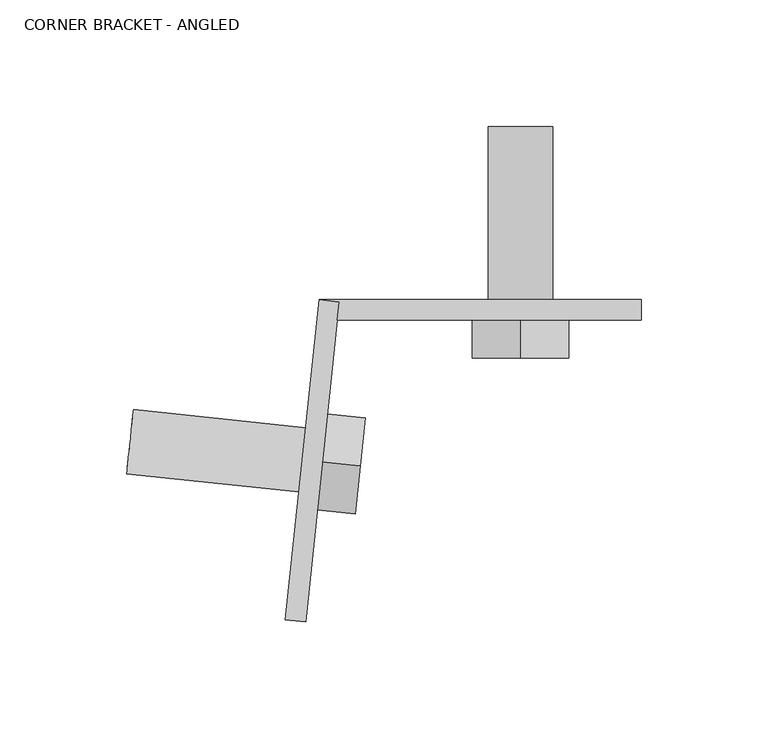
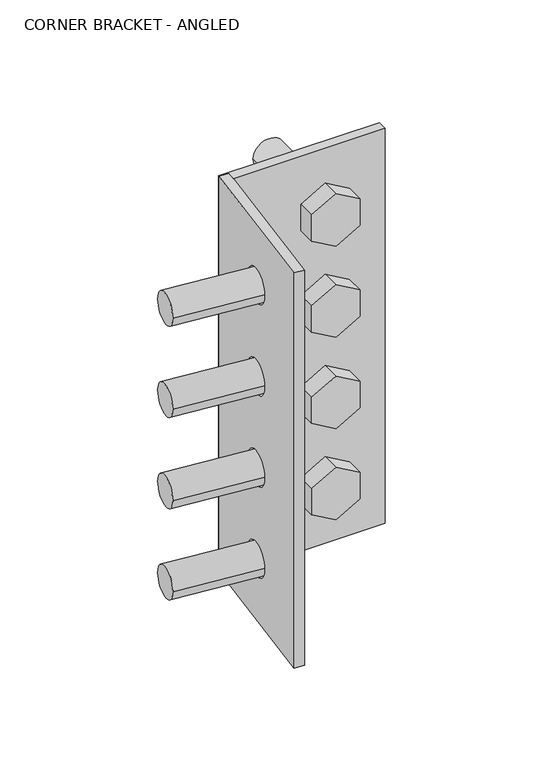
"""IFC4 building model written with IfcOpenShell, lengths in millimetres: fastener geometry, CORNER BRACKET - ANGLED."""

from ifc_helpers import new_model, si_unit, point, frame, frame_2d, origin, place, context, project, spatial, polyline, circle_curve, trimmed, segment, composite_curve, outline, extrude, source, transform, mapped, element, save
from ifc_brep_helpers import plane_surface, revolved_surface, advanced_brep


def corner_bracket_angled_dba65dea(model_context):
    return source(origin(), model_context, "Body", "SolidModel", [
        advanced_brep(
        [(65.484375, -7.9375, 203.2), (65.484375, 0.0, 203.2), (93.265625, 0.0, 203.2), (93.265625, -7.9375, 203.2), (93.265625, -7.9375, 279.4), (93.265625, 0.0, 279.4), (65.484375, 0.0, 279.4), (65.484375, -7.9375, 279.4), (127.0, 0.0, 0.0), (127.0, 0.0, 330.2), (127.0, -7.9375, 330.2), (127.0, -7.9375, 0.0), (65.484375, -7.9375, 127.0), (65.484375, 0.0, 127.0), (93.265625, 0.0, 127.0), (93.265625, -7.9375, 127.0), (65.484375, -7.9375, 50.8), (65.484375, 0.0, 50.8), (93.265625, 0.0, 50.8), (93.265625, -7.9375, 50.8), (7.1469571, -7.9375, 330.2), (7.1469571, -7.9375, 0.0), (0.0, 0.0, 0.0), (0.0, 0.0, 330.2), (7.8940175, -0.8296947, 330.2), (7.8940175, -0.8296947, 0.0)],
        [
            (0, 1),
            (1, 2, circle_curve(frame((79.375, 0.0, 203.2), z_axis=(0.0, 1.0, 0.0), x_axis=(-1.0000000000000002, 0.0, 0.0)), 13.890625)),
            (2, 3),
            (3, 0, circle_curve(frame((79.375, -7.9375, 203.2), z_axis=(0.0, -1.0, 0.0), x_axis=(-1.0000000000000002, 0.0, 0.0)), 13.890625)),
            (4, 5),
            (5, 6, circle_curve(frame((79.375, 0.0, 279.4), z_axis=(0.0, 1.0, 0.0), x_axis=(-1.0000000000000002, 0.0, 0.0)), 13.890625)),
            (6, 7),
            (7, 4, circle_curve(frame((79.375, -7.9375, 279.4), z_axis=(0.0, -1.0, 0.0), x_axis=(-1.0000000000000002, 0.0, 0.0)), 13.890625)),
            (8, 9),
            (9, 10),
            (10, 11),
            (11, 8),
            (6, 5, circle_curve(frame((79.375, 0.0, 279.4), z_axis=(0.0, 1.0, 0.0), x_axis=(-1.0000000000000002, 0.0, 0.0)), 13.890625)),
            (4, 7, circle_curve(frame((79.375, -7.9375, 279.4), z_axis=(0.0, -1.0, 0.0), x_axis=(-1.0000000000000002, 0.0, 0.0)), 13.890625)),
            (12, 13),
            (13, 14, circle_curve(frame((79.375, 0.0, 127.0), z_axis=(0.0, 1.0, 0.0), x_axis=(-1.0000000000000002, 0.0, 0.0)), 13.890625)),
            (14, 15),
            (15, 12, circle_curve(frame((79.375, -7.9375, 127.0), z_axis=(0.0, -1.0, 0.0), x_axis=(-1.0000000000000002, 0.0, 0.0)), 13.890625)),
            (16, 17),
            (17, 18, circle_curve(frame((79.375, 0.0, 50.8), z_axis=(0.0, 1.0, 0.0), x_axis=(-1.0000000000000002, 0.0, 0.0)), 13.890625)),
            (18, 19),
            (19, 16, circle_curve(frame((79.375, -7.9375, 50.8), z_axis=(0.0, -1.0, 0.0), x_axis=(-1.0000000000000002, 0.0, 0.0)), 13.890625)),
            (10, 20),
            (20, 21),
            (21, 11),
            (3, 0, circle_curve(frame((79.375, -7.9375, 203.2), z_axis=(0.0, 1.0, 0.0), x_axis=(-1.0000000000000002, 0.0, 0.0)), 13.890625)),
            (15, 12, circle_curve(frame((79.375, -7.9375, 127.0), z_axis=(0.0, 1.0, 0.0), x_axis=(-1.0000000000000002, 0.0, 0.0)), 13.890625)),
            (19, 16, circle_curve(frame((79.375, -7.9375, 50.8), z_axis=(0.0, 1.0, 0.0), x_axis=(-1.0000000000000002, 0.0, 0.0)), 13.890625)),
            (8, 22),
            (22, 23),
            (23, 9),
            (1, 2, circle_curve(frame((79.375, 0.0, 203.2), z_axis=(0.0, -1.0, 0.0), x_axis=(-1.0000000000000002, 0.0, 0.0)), 13.890625)),
            (13, 14, circle_curve(frame((79.375, 0.0, 127.0), z_axis=(0.0, -1.0, 0.0), x_axis=(-1.0000000000000002, 0.0, 0.0)), 13.890625)),
            (17, 18, circle_curve(frame((79.375, 0.0, 50.8), z_axis=(0.0, -1.0, 0.0), x_axis=(-1.0000000000000002, 0.0, 0.0)), 13.890625)),
            (23, 24),
            (24, 20),
            (21, 25),
            (25, 22),
            (24, 25),
        ],
        [
            revolved_surface(polyline([(65.484375, -7.937500000000007, 203.2), (65.484375, 0.0, 203.2)]), (79.375, 0.0, 203.2), (0.0, -1.0000000000000004, 0.0)),
            revolved_surface(polyline([(65.484375, -7.937500000000007, 279.4), (65.484375, 0.0, 279.4)]), (79.375, 0.0, 279.4), (0.0, -1.0000000000000004, 0.0)),
            plane_surface(frame((127.0, -7.9375, 330.2), z_axis=(1.0, 0.0, 0.0), x_axis=(0.0, 1.0, 0.0))),
            revolved_surface(polyline([(65.484375, -7.937500000000007, 127.0), (65.484375, 0.0, 127.0)]), (79.375, 0.0, 127.0), (0.0, -1.0000000000000004, 0.0)),
            revolved_surface(polyline([(65.484375, -7.937500000000007, 50.8), (65.484375, 0.0, 50.8)]), (79.375, 0.0, 50.8), (0.0, -1.0000000000000004, 0.0)),
            plane_surface(frame((127.0, -7.9375, 330.2), z_axis=(0.0, -1.0, 0.0), x_axis=(1.0, 0.0, 0.0))),
            plane_surface(frame((127.0, 0.0, 330.2), z_axis=(0.0, 1.0, 0.0), x_axis=(-1.0, 0.0, 0.0))),
            plane_surface(frame((0.0, -7.9375, 330.2), z_axis=(0.0, 0.0, 1.0), x_axis=(0.0, 1.0, 0.0))),
            plane_surface(frame((127.0, -7.9375, 0.0), z_axis=(0.0, 0.0, -1.0), x_axis=(0.0, 1.0, 0.0))),
            plane_surface(frame((-5.3810973, -127.1339754, 330.2), z_axis=(-0.9945218953682736, 0.10452846326765133, 0.0), x_axis=(-0.10452846326765133, -0.9945218953682736, 0.0))),
            plane_surface(frame((7.8940175, -0.8296947, 0.0), z_axis=(-0.10452846326765133, -0.9945218953682736, 0.0), x_axis=(-0.9945218953682736, 0.10452846326765133, 0.0))),
        ],
        [
            (0, [[1, 2, 3, 4]]),
            (1, [[5, 6, 7, 8]]),
            (2, [[9, 10, 11, 12]]),
            (1, [[-7, 13, -5, 14]]),
            (3, [[15, 16, 17, 18]]),
            (4, [[19, 20, 21, 22]]),
            (5, [[23, 24, 25, -11], [-14, -8], [-4, 26], [-18, 27], [-22, 28]]),
            (6, [[-9, 29, 30, 31], [-2, 32], [-16, 33], [-13, -6], [-20, 34]]),
            (7, [[35, 36, -23, -10, -31]]),
            (8, [[-25, 37, 38, -29, -12]]),
            (0, [[-3, -32, -1, -26]]),
            (3, [[-17, -33, -15, -27]]),
            (4, [[-21, -34, -19, -28]]),
            (9, [[-37, -24, -36, 39]]),
            (10, [[-35, -30, -38, -39]]),
        ],
    ),
        extrude(outline(polyline([(290.3985226, 98.425), (301.3970453, 79.375), (290.3985226, 60.325), (268.4014774, 60.325), (257.4029547, 79.375), (268.4014774, 98.425), (290.3985226, 98.425)])), frame((0.0, -22.9195312, 0.0), z_axis=(0.0, 1.0, 0.0), x_axis=(0.0, 0.0, 1.0)), (0.0, 0.0, 1.0), 14.9820312),
        extrude(outline(composite_curve([segment(trimmed(circle_curve(frame_2d((279.4, 79.375)), 12.7), [point((279.4, 92.075))], [point((279.4, 66.675))], False, "CARTESIAN"), True, "CONTINUOUS"), segment(trimmed(circle_curve(frame_2d((279.4, 79.375)), 12.7), [point((279.4, 66.675))], [point((279.4, 92.075))], False, "CARTESIAN"), True, "CONTINUOUS")], self_intersect=False)), frame((0.0, -7.9375, 0.0), z_axis=(0.0, 1.0, 0.0), x_axis=(0.0, 0.0, 1.0)), (0.0, 0.0, 1.0), 76.2),
        extrude(outline(polyline([(214.1985226, 98.425), (225.1970453, 79.375), (214.1985226, 60.325), (192.2014774, 60.325), (181.2029547, 79.375), (192.2014774, 98.425), (214.1985226, 98.425)])), frame((0.0, -22.9195312, 0.0), z_axis=(0.0, 1.0, 0.0), x_axis=(0.0, 0.0, 1.0)), (0.0, 0.0, 1.0), 14.9820312),
        extrude(outline(composite_curve([segment(trimmed(circle_curve(frame_2d((203.2, 79.375)), 12.7), [point((203.2, 92.075))], [point((203.2, 66.675))], False, "CARTESIAN"), True, "CONTINUOUS"), segment(trimmed(circle_curve(frame_2d((203.2, 79.375)), 12.7), [point((203.2, 66.675))], [point((203.2, 92.075))], False, "CARTESIAN"), True, "CONTINUOUS")], self_intersect=False)), frame((0.0, -7.9375, 0.0), z_axis=(0.0, 1.0, 0.0), x_axis=(0.0, 0.0, 1.0)), (0.0, 0.0, 1.0), 76.2),
        extrude(outline(polyline([(290.3985226, 98.425), (301.3970453, 79.375), (290.3985226, 60.325), (268.4014774, 60.325), (257.4029547, 79.375), (268.4014774, 98.425), (290.3985226, 98.425)])), frame((0.0, -22.9195312, 0.0), z_axis=(0.0, 1.0, 0.0), x_axis=(0.0, 0.0, 1.0)), (0.0, 0.0, 1.0), 14.9820312),
        extrude(outline(composite_curve([segment(trimmed(circle_curve(frame_2d((279.4, 79.375)), 12.7), [point((279.4, 92.075))], [point((279.4, 66.675))], False, "CARTESIAN"), True, "CONTINUOUS"), segment(trimmed(circle_curve(frame_2d((279.4, 79.375)), 12.7), [point((279.4, 66.675))], [point((279.4, 92.075))], False, "CARTESIAN"), True, "CONTINUOUS")], self_intersect=False)), frame((0.0, -7.9375, 0.0), z_axis=(0.0, 1.0, 0.0), x_axis=(0.0, 0.0, 1.0)), (0.0, 0.0, 1.0), 76.2),
        extrude(outline(polyline([(137.9985226, 98.425), (148.9970453, 79.375), (137.9985226, 60.325), (116.0014774, 60.325), (105.0029547, 79.375), (116.0014774, 98.425), (137.9985226, 98.425)])), frame((0.0, -22.9195312, 0.0), z_axis=(0.0, 1.0, 0.0), x_axis=(0.0, 0.0, 1.0)), (0.0, 0.0, 1.0), 14.9820312),
        extrude(outline(composite_curve([segment(trimmed(circle_curve(frame_2d((127.0, 79.375)), 12.7), [point((127.0, 92.075))], [point((127.0, 66.675))], False, "CARTESIAN"), True, "CONTINUOUS"), segment(trimmed(circle_curve(frame_2d((127.0, 79.375)), 12.7), [point((127.0, 66.675))], [point((127.0, 92.075))], False, "CARTESIAN"), True, "CONTINUOUS")], self_intersect=False)), frame((0.0, -7.9375, 0.0), z_axis=(0.0, 1.0, 0.0), x_axis=(0.0, 0.0, 1.0)), (0.0, 0.0, 1.0), 76.2),
        extrude(outline(polyline([(61.7985226, 98.425), (72.7970453, 79.375), (61.7985226, 60.325), (39.8014774, 60.325), (28.8029547, 79.375), (39.8014774, 98.425), (61.7985226, 98.425)])), frame((0.0, -22.9195312, 0.0), z_axis=(0.0, 1.0, 0.0), x_axis=(0.0, 0.0, 1.0)), (0.0, 0.0, 1.0), 14.9820312),
        extrude(outline(composite_curve([segment(trimmed(circle_curve(frame_2d((50.8, 79.375)), 12.7), [point((50.8, 92.075))], [point((50.8, 66.675))], False, "CARTESIAN"), True, "CONTINUOUS"), segment(trimmed(circle_curve(frame_2d((50.8, 79.375)), 12.7), [point((50.8, 66.675))], [point((50.8, 92.075))], False, "CARTESIAN"), True, "CONTINUOUS")], self_intersect=False)), frame((0.0, -7.9375, 0.0), z_axis=(0.0, 1.0, 0.0), x_axis=(0.0, 0.0, 1.0)), (0.0, 0.0, 1.0), 76.2),
        advanced_brep(
        [(-0.1955056, -77.7963657, 203.2), (-8.0895231, -76.9666711, 203.2), (-5.1855917, -49.3376097, 203.2), (2.7084258, -50.1673043, 203.2), (-8.0895231, -76.9666711, 279.4), (-0.1955056, -77.7963657, 279.4), (2.7084258, -50.1673043, 279.4), (-5.1855917, -49.3376097, 279.4), (-5.3810973, -127.1339754, 0.0), (-5.3810973, -127.1339754, 330.2), (-13.2751148, -126.3042807, 330.2), (-13.2751148, -126.3042807, 0.0), (-0.1955056, -77.7963657, 127.0), (-8.0895231, -76.9666711, 127.0), (-5.1855917, -49.3376097, 127.0), (2.7084258, -50.1673043, 127.0), (-0.1955056, -77.7963657, 50.8), (-8.0895231, -76.9666711, 50.8), (-5.1855917, -49.3376097, 50.8), (2.7084258, -50.1673043, 50.8), (7.8940175, -0.8296947, 330.2), (7.1469571, -7.9375, 330.2), (7.1469571, -7.9375, 0.0), (7.8940175, -0.8296947, 0.0), (0.0, 0.0, 330.2), (0.0, 0.0, 0.0)],
        [
            (0, 1),
            (1, 2, circle_curve(frame((-6.6375574, -63.1521404, 203.2), z_axis=(-0.9945218953682737, 0.10452846326765135, 0.0), x_axis=(0.10452846326765132, 0.9945218953682735, 0.0)), 13.890625)),
            (2, 3),
            (3, 0, circle_curve(frame((1.2564601, -63.981835, 203.2), z_axis=(0.9945218953682737, -0.10452846326765135, 0.0), x_axis=(0.10452846326765132, 0.9945218953682735, 0.0)), 13.890625)),
            (4, 5),
            (5, 6, circle_curve(frame((1.2564601, -63.981835, 279.4), z_axis=(0.9945218953682737, -0.10452846326765135, 0.0), x_axis=(0.10452846326765132, 0.9945218953682735, 0.0)), 13.890625)),
            (6, 7),
            (7, 4, circle_curve(frame((-6.6375574, -63.1521404, 279.4), z_axis=(-0.9945218953682737, 0.10452846326765135, 0.0), x_axis=(0.10452846326765132, 0.9945218953682735, 0.0)), 13.890625)),
            (8, 9),
            (9, 10),
            (10, 11),
            (11, 8),
            (4, 7, circle_curve(frame((-6.6375574, -63.1521404, 279.4), z_axis=(-0.9945218953682737, 0.10452846326765135, 0.0), x_axis=(0.10452846326765132, 0.9945218953682735, 0.0)), 13.890625)),
            (6, 5, circle_curve(frame((1.2564601, -63.981835, 279.4), z_axis=(0.9945218953682737, -0.10452846326765135, 0.0), x_axis=(0.10452846326765132, 0.9945218953682735, 0.0)), 13.890625)),
            (12, 13),
            (13, 14, circle_curve(frame((-6.6375574, -63.1521404, 127.0), z_axis=(-0.9945218953682737, 0.10452846326765135, 0.0), x_axis=(0.10452846326765132, 0.9945218953682735, 0.0)), 13.890625)),
            (14, 15),
            (15, 12, circle_curve(frame((1.2564601, -63.981835, 127.0), z_axis=(0.9945218953682737, -0.10452846326765135, 0.0), x_axis=(0.10452846326765132, 0.9945218953682735, 0.0)), 13.890625)),
            (16, 17),
            (17, 18, circle_curve(frame((-6.6375574, -63.1521404, 50.8), z_axis=(-0.9945218953682737, 0.10452846326765135, 0.0), x_axis=(0.10452846326765132, 0.9945218953682735, 0.0)), 13.890625)),
            (18, 19),
            (19, 16, circle_curve(frame((1.2564601, -63.981835, 50.8), z_axis=(0.9945218953682737, -0.10452846326765135, 0.0), x_axis=(0.10452846326765132, 0.9945218953682735, 0.0)), 13.890625)),
            (20, 21),
            (21, 9),
            (8, 22),
            (22, 23),
            (23, 20),
            (19, 16, circle_curve(frame((1.2564601, -63.981835, 50.8), z_axis=(-0.9945218953682737, 0.10452846326765135, 0.0), x_axis=(0.10452846326765132, 0.9945218953682735, 0.0)), 13.890625)),
            (15, 12, circle_curve(frame((1.2564601, -63.981835, 127.0), z_axis=(-0.9945218953682737, 0.10452846326765135, 0.0), x_axis=(0.10452846326765132, 0.9945218953682735, 0.0)), 13.890625)),
            (3, 0, circle_curve(frame((1.2564601, -63.981835, 203.2), z_axis=(-0.9945218953682737, 0.10452846326765135, 0.0), x_axis=(0.10452846326765132, 0.9945218953682735, 0.0)), 13.890625)),
            (24, 25),
            (25, 11),
            (10, 24),
            (1, 2, circle_curve(frame((-6.6375574, -63.1521404, 203.2), z_axis=(0.9945218953682737, -0.10452846326765135, 0.0), x_axis=(0.10452846326765132, 0.9945218953682735, 0.0)), 13.890625)),
            (17, 18, circle_curve(frame((-6.6375574, -63.1521404, 50.8), z_axis=(0.9945218953682737, -0.10452846326765135, 0.0), x_axis=(0.10452846326765132, 0.9945218953682735, 0.0)), 13.890625)),
            (13, 14, circle_curve(frame((-6.6375574, -63.1521404, 127.0), z_axis=(0.9945218953682737, -0.10452846326765135, 0.0), x_axis=(0.10452846326765132, 0.9945218953682735, 0.0)), 13.890625)),
            (20, 24),
            (25, 23),
        ],
        [
            revolved_surface(polyline([(2.7084257925952384, -50.1673043704516, 203.2), (-5.1855917299787775, -49.33760969556763, 203.2)]), (-6.6375574, -63.1521404, 203.2), (0.9945218953682735, -0.10452846326765132, 0.0)),
            revolved_surface(polyline([(2.7084257925952384, -50.1673043704516, 279.4), (-5.1855917299787775, -49.33760969556763, 279.4)]), (-6.6375574, -63.1521404, 279.4), (0.9945218953682735, -0.10452846326765132, 0.0)),
            plane_surface(frame((-5.3810973, -127.1339754, 330.2), z_axis=(-0.10452846326765133, -0.9945218953682736, 0.0), x_axis=(-0.9945218953682736, 0.10452846326765133, 0.0))),
            revolved_surface(polyline([(2.7084257925952384, -50.1673043704516, 127.0), (-5.1855917299787775, -49.33760969556763, 127.0)]), (-6.6375574, -63.1521404, 127.0), (0.9945218953682735, -0.10452846326765132, 0.0)),
            revolved_surface(polyline([(2.7084257925952384, -50.1673043704516, 50.8), (-5.1855917299787775, -49.33760969556763, 50.8)]), (-6.6375574, -63.1521404, 50.8), (0.9945218953682735, -0.10452846326765132, 0.0)),
            plane_surface(frame((-5.3810973, -127.1339754, 330.2), z_axis=(0.9945218953682736, -0.10452846326765133, 0.0), x_axis=(-0.10452846326765133, -0.9945218953682736, 0.0))),
            plane_surface(frame((-13.2751148, -126.3042807, 330.2), z_axis=(-0.9945218953682736, 0.10452846326765133, 0.0), x_axis=(0.10452846326765133, 0.9945218953682736, 0.0))),
            plane_surface(frame((7.8940175, -0.8296947, 330.2), z_axis=(0.0, 0.0, 1.0000000000000002), x_axis=(-0.9945218953682736, 0.10452846326765133, 0.0))),
            plane_surface(frame((-5.3810973, -127.1339754, 0.0), z_axis=(0.0, 0.0, -1.0000000000000002), x_axis=(-0.9945218953682736, 0.10452846326765133, 0.0))),
            plane_surface(frame((7.8940175, -0.8296947, 0.0), z_axis=(0.10452846326765133, 0.9945218953682736, 0.0), x_axis=(-0.9945218953682736, 0.10452846326765133, 0.0))),
        ],
        [
            (0, [[1, 2, 3, 4]]),
            (1, [[5, 6, 7, 8]]),
            (2, [[9, 10, 11, 12]]),
            (1, [[-5, 13, -7, 14]]),
            (3, [[15, 16, 17, 18]]),
            (4, [[19, 20, 21, 22]]),
            (5, [[23, 24, -9, 25, 26, 27], [-6, -14], [28, -22], [29, -18], [30, -4]]),
            (6, [[31, 32, -11, 33], [34, -2], [35, -20], [-8, -13], [36, -16]]),
            (7, [[-24, -23, 37, -33, -10]]),
            (8, [[-26, -25, -12, -32, 38]]),
            (9, [[-27, -38, -31, -37]]),
            (0, [[-1, -30, -3, -34]]),
            (3, [[-15, -29, -17, -36]]),
            (4, [[-19, -28, -21, -35]]),
        ],
    ),
        extrude(outline(polyline([(0.0, 0.0), (21.9970452, 0.0), (32.9955679, -19.05), (21.9970452, -38.1), (0.0, -38.1), (-10.9985227, -19.05), (0.0, 0.0)])), frame((14.165151, -84.4935258, 290.3985226), z_axis=(-0.9945218953682736, 0.10452846326765133, 0.0), x_axis=(0.0, 0.0, -1.0)), (0.0, 0.0, 1.0), 14.9820312),
        extrude(outline(composite_curve([segment(trimmed(circle_curve(frame_2d((0.0, -12.6999999)), 12.7), [point((0.0, -25.4))], [point((0.0, 0.0))], False, "CARTESIAN"), True, "CONTINUOUS"), segment(trimmed(circle_curve(frame_2d((0.0, -12.6999999)), 12.7), [point((0.0, 0.0))], [point((0.0, -25.4))], False, "CARTESIAN"), True, "CONTINUOUS")], self_intersect=False)), frame((2.5839716, -51.351407, 279.4), z_axis=(-0.9945218953682736, 0.10452846326765133, 0.0), x_axis=(0.0, 0.0, 1.0)), (0.0, 0.0, 1.0), 76.2),
        extrude(outline(polyline([(0.0, 0.0), (21.9970452, 0.0), (32.9955679, -19.05), (21.9970452, -38.1), (0.0, -38.1), (-10.9985227, -19.05), (0.0, 0.0)])), frame((14.165151, -84.4935258, 214.1985226), z_axis=(-0.9945218953682736, 0.10452846326765133, 0.0), x_axis=(0.0, 0.0, -1.0)), (0.0, 0.0, 1.0), 14.9820312),
        extrude(outline(composite_curve([segment(trimmed(circle_curve(frame_2d((0.0, -12.6999999)), 12.7), [point((0.0, -25.4))], [point((0.0, 0.0))], False, "CARTESIAN"), True, "CONTINUOUS"), segment(trimmed(circle_curve(frame_2d((0.0, -12.6999999)), 12.7), [point((0.0, 0.0))], [point((0.0, -25.4))], False, "CARTESIAN"), True, "CONTINUOUS")], self_intersect=False)), frame((2.5839716, -51.351407, 203.2), z_axis=(-0.9945218953682736, 0.10452846326765133, 0.0), x_axis=(0.0, 0.0, 1.0)), (0.0, 0.0, 1.0), 76.2),
        extrude(outline(polyline([(0.0, 0.0), (21.9970452, 0.0), (32.9955679, -19.05), (21.9970452, -38.1), (0.0, -38.1), (-10.9985227, -19.05), (0.0, 0.0)])), frame((14.165151, -84.4935258, 290.3985226), z_axis=(-0.9945218953682736, 0.10452846326765133, 0.0), x_axis=(0.0, 0.0, -1.0)), (0.0, 0.0, 1.0), 14.9820312),
        extrude(outline(composite_curve([segment(trimmed(circle_curve(frame_2d((0.0, -12.6999999)), 12.7), [point((0.0, -25.4))], [point((0.0, 0.0))], False, "CARTESIAN"), True, "CONTINUOUS"), segment(trimmed(circle_curve(frame_2d((0.0, -12.6999999)), 12.7), [point((0.0, 0.0))], [point((0.0, -25.4))], False, "CARTESIAN"), True, "CONTINUOUS")], self_intersect=False)), frame((2.5839716, -51.351407, 279.4), z_axis=(-0.9945218953682736, 0.10452846326765133, 0.0), x_axis=(0.0, 0.0, 1.0)), (0.0, 0.0, 1.0), 76.2),
        extrude(outline(polyline([(0.0, 0.0), (21.9970452, 0.0), (32.9955679, -19.05), (21.9970452, -38.1), (0.0, -38.1), (-10.9985227, -19.05), (0.0, 0.0)])), frame((14.165151, -84.4935258, 137.9985226), z_axis=(-0.9945218953682736, 0.10452846326765133, 0.0), x_axis=(0.0, 0.0, -1.0)), (0.0, 0.0, 1.0), 14.9820312),
        extrude(outline(composite_curve([segment(trimmed(circle_curve(frame_2d((0.0, -12.6999999)), 12.7), [point((0.0, -25.4))], [point((0.0, 0.0))], False, "CARTESIAN"), True, "CONTINUOUS"), segment(trimmed(circle_curve(frame_2d((0.0, -12.6999999)), 12.7), [point((0.0, 0.0))], [point((0.0, -25.4))], False, "CARTESIAN"), True, "CONTINUOUS")], self_intersect=False)), frame((2.5839716, -51.351407, 127.0), z_axis=(-0.9945218953682736, 0.10452846326765133, 0.0), x_axis=(0.0, 0.0, 1.0)), (0.0, 0.0, 1.0), 76.2),
        extrude(outline(polyline([(0.0, 0.0), (21.9970452, 0.0), (32.9955679, -19.05), (21.9970452, -38.1), (0.0, -38.1), (-10.9985227, -19.05), (0.0, 0.0)])), frame((14.165151, -84.4935258, 61.7985226), z_axis=(-0.9945218953682736, 0.10452846326765133, 0.0), x_axis=(0.0, 0.0, -1.0)), (0.0, 0.0, 1.0), 14.9820312),
        extrude(outline(composite_curve([segment(trimmed(circle_curve(frame_2d((0.0, -12.6999999)), 12.7), [point((0.0, -25.4))], [point((0.0, 0.0))], False, "CARTESIAN"), True, "CONTINUOUS"), segment(trimmed(circle_curve(frame_2d((0.0, -12.6999999)), 12.7), [point((0.0, 0.0))], [point((0.0, -25.4))], False, "CARTESIAN"), True, "CONTINUOUS")], self_intersect=False)), frame((2.5839716, -51.351407, 50.8), z_axis=(-0.9945218953682736, 0.10452846326765133, 0.0), x_axis=(0.0, 0.0, 1.0)), (0.0, 0.0, 1.0), 76.2),
    ])


if __name__ == "__main__":
    model = new_model("IFC4")
    model_context = context("Model", 3, world=origin())
    ifc_project = project(units=[si_unit("LENGTHUNIT", "METRE", prefix="MILLI")], contexts=[model_context])
    site = spatial("IfcSite", under=ifc_project)
    building = spatial("IfcBuilding", under=site)
    placement = place(None, origin())
    corner_bracket_angled_shape = corner_bracket_angled_dba65dea(model_context)
    element("IfcFastener", 1, ObjectType="CORNER BRACKET - ANGLED : CUSTOM - L5\"x5\"x5/16\"x13\" (BENT ANGLE - 96°) - HDG", at=placement, inside=building, context=model_context, shape_type="MappedRepresentation", body=[
        mapped(corner_bracket_angled_shape, transform((0.0, 0.0, 0.0), x_axis=(1.0, 0.0, 0.0), y_axis=(0.0, 1.0, 0.0), z_axis=(0.0, 0.0, 1.0))),
    ])
    save(model, "model.ifc")

# Revit data of these elements
# Type "CORNER BRACKET - ANGLED : CUSTOM - L5\"x5\"x5/16\"x13\" (BENT ANGLE - 96°) - HDG"
#   URL = "https://www.strongtie.com/classiccollection_architecturalproductsgroup/hlpc-hlgpc_productgroup_wcc/p/hlpc.hlgpc"
#   Default Elevation = 4' - 0"
#   Angle = 96.00°
#   Leg Two = element 1900782
#   Leg One = element 1905931
#   URL = ""
# Element 1 (IfcFastener, "CORNER BRACKET - ANGLED : CUSTOM - L5\"x5\"x5/16\"x13\" (BENT ANGLE - 96°) - HDG")
#   Materials on its faces: "1\" GALV. LAG BOLT (LENGTH = 1/2\" SHY OF GLULAM DEPTH) -  (GALV. THRU BOLT IF PLATE ON OPP. SIDE OF STRUCT MEMBER)", "L5\"x5\"x5/16\" STEEL ANGLE (HDG AFTER FABRICATION)"
# Materials
#   "1\" GALV. LAG BOLT (LENGTH = 1/2\" SHY OF GLULAM DEPTH) -  (GALV. THRU BOLT IF PLATE ON OPP. SIDE OF STRUCT MEMBER)": class "Generic", colour RGB 120 120 120, transparency 0, Cost = 0
#   "L5\"x5\"x5/16\" STEEL ANGLE (HDG AFTER FABRICATION)": class "Generic", colour RGB 232 232 232, transparency 0, Cost = 0
